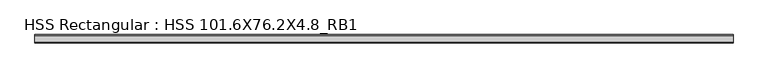
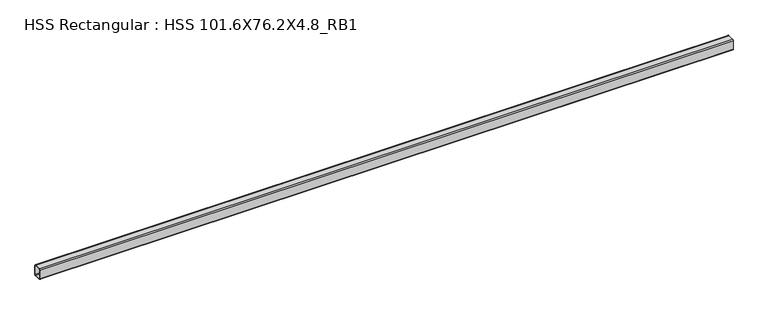
"""IFC4 building model written with IfcOpenShell, lengths in millimetres: beam geometry, HSS Rectangular : HSS 101.6X76.2X4.8_RB1."""

from ifc_helpers import new_model, si_unit, point, frame, frame_2d, origin, place, context, project, spatial, polyline, circle_curve, trimmed, segment, composite_curve, outline, extrude, source, transform, mapped, element, save


def hss_rectangular_hss_101_6x76_2x4_8_rb1_df45e8b3(model_context):
    return source(origin(), model_context, "Body", "SweptSolid", [
        extrude(outline(composite_curve([segment(polyline([(38.1, 41.275), (38.1, -41.275)]), True, "CONTINUOUS"), segment(trimmed(circle_curve(frame_2d((28.575, -41.275)), 9.525), [point((38.1, -41.275))], [point((28.575, -50.8))], False, "CARTESIAN"), True, "CONTINUOUS"), segment(polyline([(28.575, -50.8), (-28.575, -50.8)]), True, "CONTINUOUS"), segment(trimmed(circle_curve(frame_2d((-28.575, -41.275)), 9.525), [point((-28.575, -50.8))], [point((-38.1, -41.275))], False, "CARTESIAN"), True, "CONTINUOUS"), segment(polyline([(-38.1, -41.275), (-38.1, 41.275)]), True, "CONTINUOUS"), segment(trimmed(circle_curve(frame_2d((-28.575, 41.275)), 9.525), [point((-38.1, 41.275))], [point((-28.575, 50.8))], False, "CARTESIAN"), True, "CONTINUOUS"), segment(polyline([(-28.575, 50.8), (28.575, 50.8)]), True, "CONTINUOUS"), segment(trimmed(circle_curve(frame_2d((28.575, 41.275)), 9.525), [point((28.575, 50.8))], [point((38.1, 41.275))], False, "CARTESIAN"), True, "CONTINUOUS")], self_intersect=False), holes=[composite_curve([segment(trimmed(circle_curve(frame_2d((-28.575, 41.275)), 4.7625), [point((-28.575, 46.0375))], [point((-33.3375, 41.275))], True, "CARTESIAN"), True, "CONTINUOUS"), segment(polyline([(-33.3375, 41.275), (-33.3375, -41.275)]), True, "CONTINUOUS"), segment(trimmed(circle_curve(frame_2d((-28.575, -41.275)), 4.7625), [point((-33.3375, -41.275))], [point((-28.575, -46.0375))], True, "CARTESIAN"), True, "CONTINUOUS"), segment(polyline([(-28.575, -46.0375), (28.575, -46.0375)]), True, "CONTINUOUS"), segment(trimmed(circle_curve(frame_2d((28.575, -41.275)), 4.7625), [point((28.575, -46.0375))], [point((33.3375, -41.275))], True, "CARTESIAN"), True, "CONTINUOUS"), segment(polyline([(33.3375, -41.275), (33.3375, 41.275)]), True, "CONTINUOUS"), segment(trimmed(circle_curve(frame_2d((28.575, 41.275)), 4.7625), [point((33.3375, 41.275))], [point((28.575, 46.0375))], True, "CARTESIAN"), True, "CONTINUOUS"), segment(polyline([(28.575, 46.0375), (-28.575, 46.0375)]), True, "CONTINUOUS")], self_intersect=False)]), frame((-7634.3387302, 0.0, 0.0), z_axis=(1.0, 0.0, 0.0), x_axis=(0.0, 1.0, 0.0)), (0.0, 0.0, 1.0), 6300.0877191),
    ])


if __name__ == "__main__":
    model = new_model("IFC4")
    model_context = context("Model", 3, world=origin())
    ifc_project = project(units=[si_unit("LENGTHUNIT", "METRE", prefix="MILLI")], contexts=[model_context])
    site = spatial("IfcSite", under=ifc_project)
    building = spatial("IfcBuilding", under=site)
    placement = place(None, origin())
    hss_rectangular_hss_101_6x76_2x4_8_rb1_shape = hss_rectangular_hss_101_6x76_2x4_8_rb1_df45e8b3(model_context)
    element("IfcBeam", 1, ObjectType="HSS Rectangular : HSS 101.6X76.2X4.8_RB1", at=placement, inside=building, context=model_context, shape_type="MappedRepresentation", body=[
        mapped(hss_rectangular_hss_101_6x76_2x4_8_rb1_shape, transform((0.0, 0.0, 0.0), x_axis=(1.0, 0.0, 0.0), y_axis=(0.0, 1.0, 0.0), z_axis=(0.0, 0.0, 1.0))),
    ])
    save(model, "model.ifc")

# Revit data of these elements
# Type "HSS Rectangular : HSS 101.6X76.2X4.8_RB1"
#   Section Name Key = "HSS 4X3X3/16"
#   Assembly Code = "B10"
#   Width = 7.62 cm
#   Wall Nominal Thickness = 0.4763 cm
#   Wall Design Thickness = 0.442 cm
#   Torsional Moment of Inertia = 260.561 cm⁴
#   Torsional Modulus = 61.2876 cm³
#   Section Area = 14.4516 cm²
#   Plastic Modulus weak axis = 40.3122 cm³
#   Plastic Modulus strong axis = 49.1612 cm³
#   Perimeter = 0.881482 m²/m
#   Outer Fillet = 0.9525 cm
#   Nominal Weight = 12.1285 kgf/m
#   Moment of Inertia weak axis = 131.529 cm⁴
#   Moment of Inertia strong axis = 205.202 cm⁴
#   Inner Fillet = 0.4763 cm
#   Height = 10.16 cm
#   Elastic Modulus weak axis = 34.4128 cm³
#   Elastic Modulus strong axis = 40.476 cm³
#   Centroid Vertical = 5.08 cm
#   Centroid Horizontal = 3.81 cm
#   Length [instance default] = 1524 mm
#   Structural Material [instance default] = Steel ASTM A500, Grade B, Rectangular and Square
#   Principal Axes Angle = 0
# Element 1 (IfcBeam, "HSS Rectangular : HSS 101.6X76.2X4.8_RB1")
#   Structural Material = Steel ASTM A992
#   Materials on its faces: "Steel ASTM A992"
# Materials
#   "Steel ASTM A500, Grade B, Rectangular and Square": class "Metal", colour RGB 199 199 199, transparency 0, Description = "Carbon steel", Cost = 0
#   "Steel ASTM A992": class "Metal", colour RGB 199 199 199, transparency 0, Description = "Structural steel 50ksi", Cost = 0
